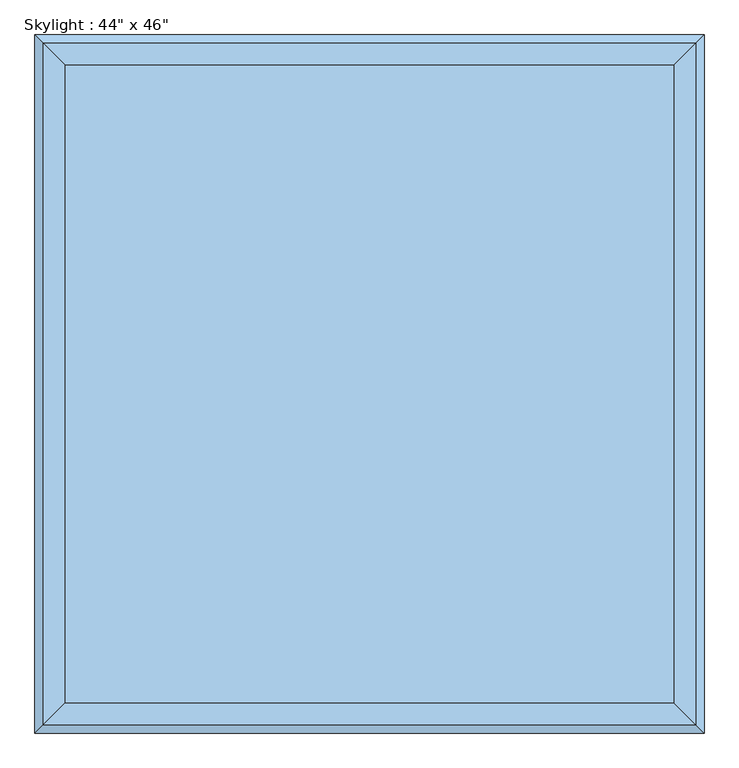
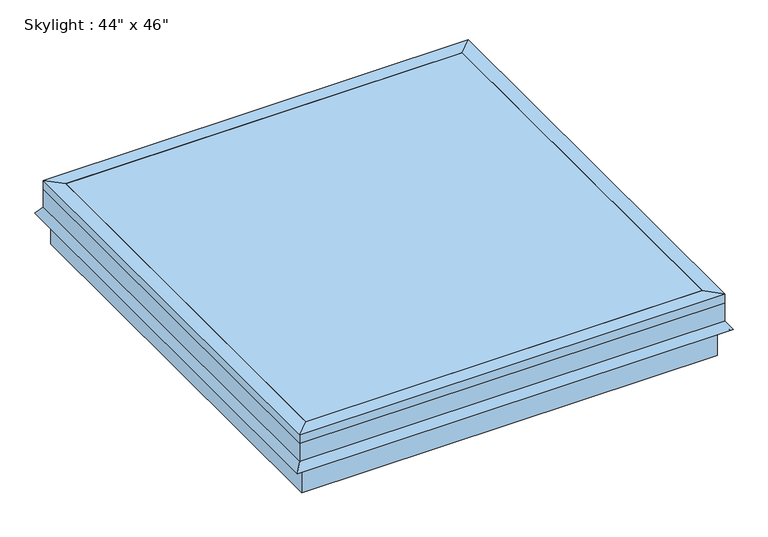
"""IFC4 building model written with IfcOpenShell, lengths in millimetres: window geometry."""

from ifc_helpers import new_model, si_unit, frame, origin, place, context, project, spatial, polyline, outline, extrude, faceted_brep, source, transform, mapped, element, save


def window_c0717641(model_context):
    return source(origin(), model_context, "Body", "SolidModel", [
        faceted_brep([(254.440073, 370.1040988, 4114.8), (279.840073, 395.5040988, 4114.8), (279.840073, -772.8959012, 4114.8), (254.440073, -747.4959012, 4114.8), (254.440073, 370.1040988, 4140.2), (254.440073, -747.4959012, 4140.2), (292.540073, 408.2040988, 4140.2), (292.540073, -785.5959012, 4140.2), (292.540073, 408.2040988, 4114.8), (292.540073, -785.5959012, 4114.8), (292.540073, 408.2040988, 4064.0), (292.540073, -785.5959012, 4064.0), (307.1089145, 422.7729403, 4043.1935381), (307.1089145, -800.1647427, 4043.1935381), (301.907299, 417.5713248, 4039.5513277), (301.907299, -794.9631272, 4039.5513277), (286.190073, 401.8540988, 4061.9978527), (286.190073, -779.2459012, 4061.9978527), (286.190073, 401.8540988, 4114.8), (286.190073, -779.2459012, 4114.8), (-837.759927, -772.8959012, 4114.8), (-812.359927, -747.4959012, 4114.8), (-812.359927, -747.4959012, 4140.2), (-850.459927, -785.5959012, 4140.2), (-850.459927, -785.5959012, 4114.8), (-850.459927, -785.5959012, 4064.0), (-865.0287685, -800.1647427, 4043.1935381), (-859.827153, -794.9631272, 4039.5513277), (-844.109927, -779.2459012, 4061.9978527), (-844.109927, -779.2459012, 4114.8), (-837.759927, 395.5040988, 4114.8), (-812.359927, 370.1040988, 4114.8), (-812.359927, 370.1040988, 4140.2), (-850.459927, 408.2040988, 4140.2), (-850.459927, 408.2040988, 4114.8), (-850.459927, 408.2040988, 4064.0), (-865.0287685, 422.7729403, 4043.1935381), (-859.827153, 417.5713248, 4039.5513277), (-844.109927, 401.8540988, 4061.9978527), (-844.109927, 401.8540988, 4114.8)], [[[0, 1, 2, 3]], [[4, 0, 3, 5]], [[6, 4, 5, 7]], [[8, 6, 7, 9]], [[10, 8, 9, 11]], [[12, 10, 11, 13]], [[14, 12, 13, 15]], [[16, 14, 15, 17]], [[18, 16, 17, 19]], [[1, 18, 19, 2]], [[3, 2, 20, 21]], [[5, 3, 21, 22]], [[7, 5, 22, 23]], [[9, 7, 23, 24]], [[11, 9, 24, 25]], [[13, 11, 25, 26]], [[15, 13, 26, 27]], [[17, 15, 27, 28]], [[19, 17, 28, 29]], [[2, 19, 29, 20]], [[21, 20, 30, 31]], [[22, 21, 31, 32]], [[23, 22, 32, 33]], [[24, 23, 33, 34]], [[25, 24, 34, 35]], [[26, 25, 35, 36]], [[27, 26, 36, 37]], [[28, 27, 37, 38]], [[29, 28, 38, 39]], [[20, 29, 39, 30]], [[31, 30, 1, 0]], [[32, 31, 0, 4]], [[33, 32, 4, 6]], [[34, 33, 6, 8]], [[35, 34, 8, 10]], [[36, 35, 10, 12]], [[37, 36, 12, 14]], [[38, 37, 14, 16]], [[39, 38, 16, 18]], [[30, 39, 18, 1]]]),
        faceted_brep([(279.840073, -772.8959012, 4114.8), (279.840073, -772.8959012, 3962.4), (279.840073, 395.5040988, 3962.4), (279.840073, 395.5040988, 4114.8), (254.440073, -747.4959012, 4114.8), (254.440073, 370.1040988, 4114.8), (254.440073, -747.4959012, 4089.4), (254.440073, 370.1040988, 4089.4), (235.390073, -728.4459012, 4089.4), (235.390073, 351.0540988, 4089.4), (235.390073, -728.4459012, 3962.4), (235.390073, 351.0540988, 3962.4), (-837.759927, 395.5040988, 3962.4), (-837.759927, 395.5040988, 4114.8), (-812.359927, 370.1040988, 4114.8), (-812.359927, 370.1040988, 4089.4), (-793.309927, 351.0540988, 4089.4), (-793.309927, 351.0540988, 3962.4), (-837.759927, -772.8959012, 3962.4), (-837.759927, -772.8959012, 4114.8), (-812.359927, -747.4959012, 4114.8), (-812.359927, -747.4959012, 4089.4), (-793.309927, -728.4459012, 4089.4), (-793.309927, -728.4459012, 3962.4)], [[[0, 1, 2, 3]], [[4, 0, 3, 5]], [[6, 4, 5, 7]], [[8, 6, 7, 9]], [[10, 8, 9, 11]], [[1, 10, 11, 2]], [[3, 2, 12, 13]], [[5, 3, 13, 14]], [[7, 5, 14, 15]], [[9, 7, 15, 16]], [[11, 9, 16, 17]], [[2, 11, 17, 12]], [[13, 12, 18, 19]], [[14, 13, 19, 20]], [[15, 14, 20, 21]], [[16, 15, 21, 22]], [[17, 16, 22, 23]], [[12, 17, 23, 18]], [[19, 18, 1, 0]], [[20, 19, 0, 4]], [[21, 20, 4, 6]], [[22, 21, 6, 8]], [[23, 22, 8, 10]], [[18, 23, 10, 1]]]),
        extrude(outline(polyline([(254.440073, -747.4959012), (-812.359927, -747.4959012), (-812.359927, 370.1040988), (254.440073, 370.1040988), (254.440073, -747.4959012)])), frame((0.0, 0.0, 4133.85), z_axis=(0.0, 0.0, 1.0), x_axis=(1.0, 0.0, 0.0)), (0.0, 0.0, 1.0), 6.35),
    ])


if __name__ == "__main__":
    model = new_model("IFC4")
    model_context = context("Model", 3, world=origin())
    ifc_project = project(units=[si_unit("LENGTHUNIT", "METRE", prefix="MILLI")], contexts=[model_context])
    site = spatial("IfcSite", under=ifc_project)
    building = spatial("IfcBuilding", under=site)
    placement = place(None, origin())
    window_shape = window_c0717641(model_context)
    element("IfcWindow", 1, ObjectType="Skylight : 44\" x 46\"", at=placement, inside=building, context=model_context, shape_type="MappedRepresentation", body=[
        mapped(window_shape, transform((0.0, 0.0, 0.0), x_axis=(1.0, 0.0, 0.0), y_axis=(0.0, 1.0, 0.0), z_axis=(0.0, 0.0, 1.0))),
    ])
    save(model, "model.ifc")

# Revit data of these elements
# Type "Skylight : 44\" x 46\""
#   Type Mark = "50"
#   Construction Type Id = "GSP4R"
#   Assembly Code = "B3020110"
#   Analytic Construction = "1/8 in Pilkington single glazing"
#   Visual Light Transmittance = 0.9
#   Solar Heat Gain Coefficient = 0.78
#   Heat Transfer Coefficient (U) = 3.6886 W/(m²·K)
#   Height = 1168.4 mm
#   Width = 1117.6 mm
#   Glass Pane = Glass
#   Frame Material = Metal - Bronze, Light Brush
#   Type Comments = ""
# Element 1 (IfcWindow, "Skylight : 44\" x 46\"")
#   Materials on its faces: "Metal - Bronze, Light Brush", "Glass"
# Materials
#   "Glass": class "Glass", colour RGB 0 128 192, transparency 0.9, Description = "Soda Lime Glass", Cost = 0
#   "Metal - Bronze, Light Brush": class "Metal", colour RGB 113 80 70, transparency 0
